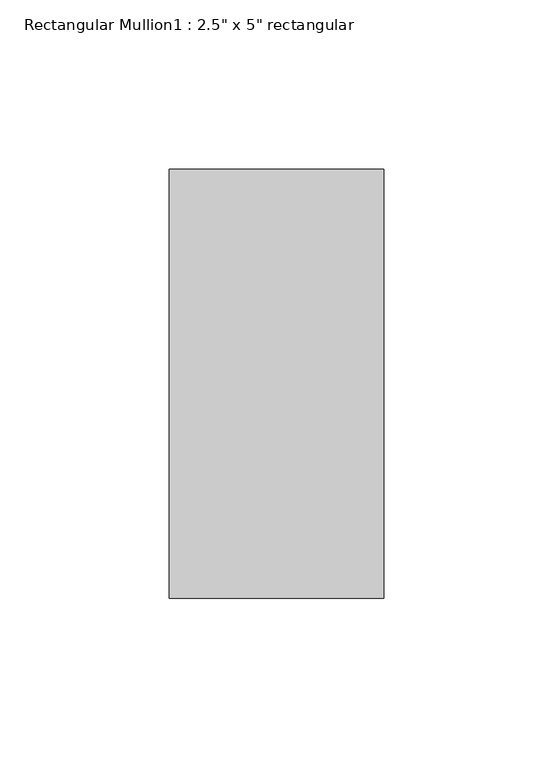
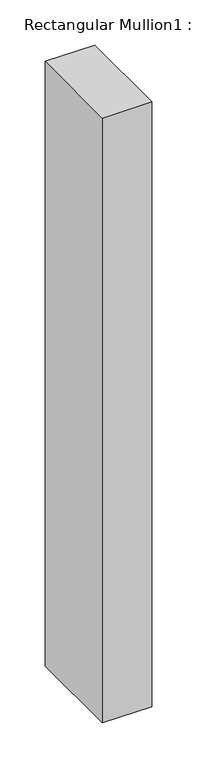
"""IFC4 building model written with IfcOpenShell, lengths in millimetres: member geometry."""

import ifcopenshell
import ifcopenshell.guid

model = None  # the IFC model being written
_history = None  # IfcOwnerHistory: only IFC2X3 demands one
_inside = {}  # id of a spatial element -> (the spatial element, [elements in it])
_under = {}  # id of a project, library or spatial element -> (it, [spatial elements below it])
_declared = {}  # id of a project -> (the project, [libraries it declares])
_typed = {}  # id of a type object -> (the type object, [elements of that type])
_made_of = {}  # id of a material, layer set ... -> (it, [elements and type objects made of it])


def new_model(schema):
    """Start an empty IFC model of exactly this schema.

    Asked for "IFC4X3", IfcOpenShell would pick the latest addendum, in which some entities
    have other attributes; the version numbers below select the first issue.
    IFC2X3 requires an IfcOwnerHistory on every rooted entity: one is made here for all.
    """
    global model, _history
    if schema == "IFC4X3":
        model = ifcopenshell.file(schema_version=(4, 3, 0, 0))
    else:
        model = ifcopenshell.file(schema=schema)
    _inside.clear()
    _under.clear()
    _declared.clear()
    _typed.clear()
    _made_of.clear()
    _history = None
    if model.schema == "IFC2X3":
        org = make("IfcOrganization", Name="unknown")
        user = make(
            "IfcPersonAndOrganization",
            ThePerson=make("IfcPerson", FamilyName="unknown"),
            TheOrganization=org,
        )
        app = make(
            "IfcApplication",
            ApplicationDeveloper=org,
            Version="unknown",
            ApplicationFullName="unknown",
            ApplicationIdentifier="unknown",
        )
        _history = make(
            "IfcOwnerHistory",
            OwningUser=user,
            OwningApplication=app,
            ChangeAction="ADDED",
            CreationDate=0,
        )
    return model


def make(cls, **values):
    """One entity of the class cls with the attributes given. An attribute that is None is left unset."""
    return model.create_entity(
        cls, **{name: value for name, value in values.items() if value is not None}
    )


def rooted(cls, **values):
    """An entity with a GlobalId (a new one), such as an element, a storey or a relation."""
    return make(cls, GlobalId=ifcopenshell.guid.new(), OwnerHistory=_history, **values)


def si_unit(unit_type, name, prefix=None):
    """IfcSIUnit, for example si_unit("LENGTHUNIT", "METRE", prefix="MILLI")."""
    return make("IfcSIUnit", UnitType=unit_type, Prefix=prefix, Name=name)


def assignment(units):
    """IfcUnitAssignment: the units of a project."""
    return None if units is None else make("IfcUnitAssignment", Units=units)


def point(xyz):
    """IfcCartesianPoint."""
    return None if xyz is None else make("IfcCartesianPoint", Coordinates=xyz)


def direction(xyz):
    """IfcDirection."""
    return None if xyz is None else make("IfcDirection", DirectionRatios=xyz)


def frame(location, z_axis=None, x_axis=None):
    """IfcAxis2Placement3D, a coordinate frame: its origin and axes. An axis left out is left unset."""
    return make(
        "IfcAxis2Placement3D",
        Location=point(location),
        Axis=direction(z_axis),
        RefDirection=direction(x_axis),
    )


def origin():
    """The frame at (0, 0, 0) with its axes left unset."""
    return frame((0.0, 0.0, 0.0))


def place(relative_to, where):
    """IfcLocalPlacement: puts the frame where relative to a parent placement (None: the world)."""
    return make(
        "IfcLocalPlacement", PlacementRelTo=relative_to, RelativePlacement=where
    )


def context(
    kind, dimensions, precision=None, world=None, true_north=None, identifier=None
):
    """IfcGeometricRepresentationContext, for example the 3D "Model" context."""
    return make(
        "IfcGeometricRepresentationContext",
        ContextIdentifier=identifier,
        ContextType=kind,
        CoordinateSpaceDimension=dimensions,
        Precision=precision,
        WorldCoordinateSystem=world,
        TrueNorth=true_north,
    )


def project(units=None, contexts=None):
    """IfcProject with its units and contexts."""
    return rooted(
        "IfcProject",
        Name="project",
        RepresentationContexts=contexts,
        UnitsInContext=assignment(units),
    )


def spatial(cls, under=None, at=None, **own):
    """A site, building, storey or space (cls), placed at a placement, below another one or the project."""
    s = rooted(cls, ObjectPlacement=at, **own)
    if under is not None:
        _under.setdefault(under.id(), (under, []))[1].append(s)
    return s


def polyline(points):
    """IfcPolyline through the points."""
    return make("IfcPolyline", Points=[point(p) for p in points])


def outline(outer, holes=None, kind="AREA"):
    """IfcArbitraryClosedProfileDef: a profile drawn as a closed curve; with holes, ...WithVoids."""
    if holes is None:
        return make("IfcArbitraryClosedProfileDef", ProfileType=kind, OuterCurve=outer)
    return make(
        "IfcArbitraryProfileDefWithVoids",
        ProfileType=kind,
        OuterCurve=outer,
        InnerCurves=holes,
    )


def extrude(swept, where, along, depth):
    """IfcExtrudedAreaSolid: the profile swept, set in the frame where, extruded along a direction by depth."""
    return make(
        "IfcExtrudedAreaSolid",
        SweptArea=swept,
        Position=where,
        ExtrudedDirection=direction(along),
        Depth=depth,
    )


def shape(context_of_items, identifier, shape_type, items):
    """IfcShapeRepresentation: the items that make up one representation, for example the "Body"."""
    return make(
        "IfcShapeRepresentation",
        ContextOfItems=context_of_items,
        RepresentationIdentifier=identifier,
        RepresentationType=shape_type,
        Items=items,
    )


def source(mapping_origin, context_of_items, identifier, shape_type, items):
    """IfcRepresentationMap: a shape defined once, which mapped items show again and again."""
    return make(
        "IfcRepresentationMap",
        MappingOrigin=mapping_origin,
        MappedRepresentation=shape(context_of_items, identifier, shape_type, items),
    )


def transform(
    local_origin,
    x_axis=None,
    y_axis=None,
    z_axis=None,
    scale=None,
    scale2=None,
    scale3=None,
    uniform=True,
):
    """IfcCartesianTransformationOperator3D, or its non-uniform kind. x_axis, y_axis, z_axis: its Axis1, 2, 3."""
    if uniform:
        return make(
            "IfcCartesianTransformationOperator3D",
            Axis1=direction(x_axis),
            Axis2=direction(y_axis),
            LocalOrigin=point(local_origin),
            Scale=scale,
            Axis3=direction(z_axis),
        )
    return make(
        "IfcCartesianTransformationOperator3DnonUniform",
        Axis1=direction(x_axis),
        Axis2=direction(y_axis),
        LocalOrigin=point(local_origin),
        Scale=scale,
        Axis3=direction(z_axis),
        Scale2=scale2,
        Scale3=scale3,
    )


def mapped(mapping_source, mapping_target):
    """IfcMappedItem: shows the shape of a source again, moved by a transform."""
    return make(
        "IfcMappedItem", MappingSource=mapping_source, MappingTarget=mapping_target
    )


def made_of(thing, what):
    """Note that an element or type object is made of a material, layer set ...; save() writes the relation."""
    if what is not None:
        _made_of.setdefault(what.id(), (what, []))[1].append(thing)
    return thing


def element(
    cls,
    number,
    at=None,
    inside=None,
    cuts=None,
    type_object=None,
    material=None,
    context=None,
    identifier="Body",
    shape_type=None,
    held_by="IfcProductDefinitionShape",
    body=None,
    shapes=None,
    **own,
):
    """One element of the class cls, such as IfcWall. Its Tag is "e" and its number.

    at: its placement. inside: the storey or other place that contains it. cuts: it is an
    opening in that element (IfcRelVoidsElement). A single representation is given by context,
    identifier, shape_type and body (its items); several are given by shapes. held_by: the class
    of the entity that holds the representations. save() writes the other relations.
    """
    e = rooted(cls, Tag="e%d" % number, ObjectPlacement=at, **own)
    if body is not None:
        shapes = [shape(context, identifier, shape_type, body)]
    if shapes is not None:
        e.Representation = make(held_by, Representations=shapes)
    if inside is not None:
        _inside.setdefault(inside.id(), (inside, []))[1].append(e)
    if cuts is not None:
        rooted(
            "IfcRelVoidsElement", RelatingBuildingElement=cuts, RelatedOpeningElement=e
        )
    if type_object is not None:
        _typed.setdefault(type_object.id(), (type_object, []))[1].append(e)
    return made_of(e, material)


def aggregate(whole, parts):
    """IfcRelAggregates: a whole, such as a stair, and the parts it consists of."""
    return rooted("IfcRelAggregates", RelatingObject=whole, RelatedObjects=parts)


def save(model, path):
    """Write the relations noted so far, then the file.

    IfcRelAggregates (storeys below a building ...), IfcRelContainedInSpatialStructure (elements
    in a storey), IfcRelDefinesByType, IfcRelAssociatesMaterial and IfcRelDeclares: one each for
    every whole, place, type object, material and project.
    """
    for whole, parts in _under.values():
        aggregate(whole, parts)
    for where, things in _inside.values():
        rooted(
            "IfcRelContainedInSpatialStructure",
            RelatedElements=things,
            RelatingStructure=where,
        )
    for kind, things in _typed.values():
        rooted("IfcRelDefinesByType", RelatedObjects=things, RelatingType=kind)
    for what, things in _made_of.values():
        rooted("IfcRelAssociatesMaterial", RelatedObjects=things, RelatingMaterial=what)
    for by, libraries in _declared.values():
        rooted("IfcRelDeclares", RelatingContext=by, RelatedDefinitions=libraries)
    model.write(path)


def member_c17f1be2(model_context):
    return source(origin(), model_context, "Body", "SweptSolid", [
        extrude(outline(polyline([(0.0, 63.5), (0.0, -63.5), (-63.5, -63.5), (-63.5, 63.5), (0.0, 63.5)])), frame((0.0, 0.0, -819.15), z_axis=(0.0, 0.0, 1.0), x_axis=(1.0, 0.0, 0.0)), (0.0, 0.0, 1.0), 819.15),
    ])


if __name__ == "__main__":
    model = new_model("IFC4")
    model_context = context("Model", 3, world=origin())
    ifc_project = project(units=[si_unit("LENGTHUNIT", "METRE", prefix="MILLI")], contexts=[model_context])
    site = spatial("IfcSite", under=ifc_project)
    building = spatial("IfcBuilding", under=site)
    placement = place(None, origin())
    member_shape = member_c17f1be2(model_context)
    element("IfcMember", 1, ObjectType="Rectangular Mullion1 : 2.5\" x 5\" rectangular", at=placement, inside=building, context=model_context, shape_type="MappedRepresentation", body=[
        mapped(member_shape, transform((0.0, 0.0, 0.0), x_axis=(1.0, 0.0, 0.0), y_axis=(0.0, 1.0, 0.0), z_axis=(0.0, 0.0, 1.0))),
    ])
    save(model, "model.ifc")

# Revit data of these elements
# Type "Rectangular Mullion1 : 2.5\" x 5\" rectangular"
#   built-in parameter 1007304 = 0.416667 (stored number, unit not read)
#   built-in parameter 1007301 = 0.104167 (stored number, unit not read)
#   built-in parameter 1007300 = 0.104167 (stored number, unit not read)
# Element 1 (IfcMember, "Rectangular Mullion1 : 2.5\" x 5\" rectangular")
#   Materials on its faces: "support-frame"
# Materials
#   "support-frame": class "Unassigned", colour RGB 233 233 233, transparency 0, Cost = 0
